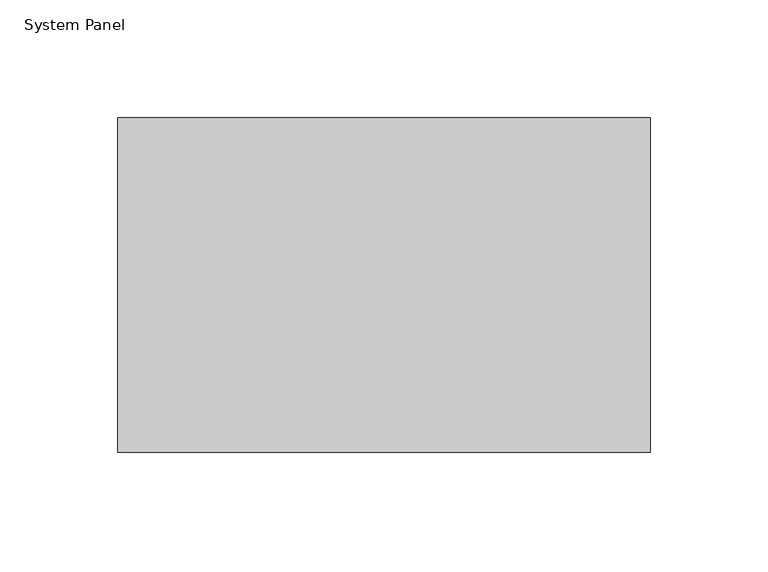
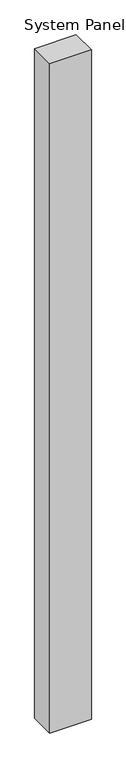
"""IFC4 building model written with IfcOpenShell, lengths in millimetres: plate geometry, System Panel : NLRS_21_CWP_hsb-vulling minerale wol 142 _gen_rsf."""

import ifcopenshell
import ifcopenshell.guid

model = None  # the IFC model being written
_history = None  # IfcOwnerHistory: only IFC2X3 demands one
_inside = {}  # id of a spatial element -> (the spatial element, [elements in it])
_under = {}  # id of a project, library or spatial element -> (it, [spatial elements below it])
_declared = {}  # id of a project -> (the project, [libraries it declares])
_typed = {}  # id of a type object -> (the type object, [elements of that type])
_made_of = {}  # id of a material, layer set ... -> (it, [elements and type objects made of it])


def new_model(schema):
    """Start an empty IFC model of exactly this schema.

    Asked for "IFC4X3", IfcOpenShell would pick the latest addendum, in which some entities
    have other attributes; the version numbers below select the first issue.
    IFC2X3 requires an IfcOwnerHistory on every rooted entity: one is made here for all.
    """
    global model, _history
    if schema == "IFC4X3":
        model = ifcopenshell.file(schema_version=(4, 3, 0, 0))
    else:
        model = ifcopenshell.file(schema=schema)
    _inside.clear()
    _under.clear()
    _declared.clear()
    _typed.clear()
    _made_of.clear()
    _history = None
    if model.schema == "IFC2X3":
        org = make("IfcOrganization", Name="unknown")
        user = make(
            "IfcPersonAndOrganization",
            ThePerson=make("IfcPerson", FamilyName="unknown"),
            TheOrganization=org,
        )
        app = make(
            "IfcApplication",
            ApplicationDeveloper=org,
            Version="unknown",
            ApplicationFullName="unknown",
            ApplicationIdentifier="unknown",
        )
        _history = make(
            "IfcOwnerHistory",
            OwningUser=user,
            OwningApplication=app,
            ChangeAction="ADDED",
            CreationDate=0,
        )
    return model


def make(cls, **values):
    """One entity of the class cls with the attributes given. An attribute that is None is left unset."""
    return model.create_entity(
        cls, **{name: value for name, value in values.items() if value is not None}
    )


def rooted(cls, **values):
    """An entity with a GlobalId (a new one), such as an element, a storey or a relation."""
    return make(cls, GlobalId=ifcopenshell.guid.new(), OwnerHistory=_history, **values)


def si_unit(unit_type, name, prefix=None):
    """IfcSIUnit, for example si_unit("LENGTHUNIT", "METRE", prefix="MILLI")."""
    return make("IfcSIUnit", UnitType=unit_type, Prefix=prefix, Name=name)


def assignment(units):
    """IfcUnitAssignment: the units of a project."""
    return None if units is None else make("IfcUnitAssignment", Units=units)


def point(xyz):
    """IfcCartesianPoint."""
    return None if xyz is None else make("IfcCartesianPoint", Coordinates=xyz)


def direction(xyz):
    """IfcDirection."""
    return None if xyz is None else make("IfcDirection", DirectionRatios=xyz)


def frame(location, z_axis=None, x_axis=None):
    """IfcAxis2Placement3D, a coordinate frame: its origin and axes. An axis left out is left unset."""
    return make(
        "IfcAxis2Placement3D",
        Location=point(location),
        Axis=direction(z_axis),
        RefDirection=direction(x_axis),
    )


def origin():
    """The frame at (0, 0, 0) with its axes left unset."""
    return frame((0.0, 0.0, 0.0))


def origin_with_axes():
    """The frame at (0, 0, 0) with the z axis (0, 0, 1) and the x axis (1, 0, 0) written out."""
    return frame((0.0, 0.0, 0.0), z_axis=(0.0, 0.0, 1.0), x_axis=(1.0, 0.0, 0.0))


def place(relative_to, where):
    """IfcLocalPlacement: puts the frame where relative to a parent placement (None: the world)."""
    return make(
        "IfcLocalPlacement", PlacementRelTo=relative_to, RelativePlacement=where
    )


def context(
    kind, dimensions, precision=None, world=None, true_north=None, identifier=None
):
    """IfcGeometricRepresentationContext, for example the 3D "Model" context."""
    return make(
        "IfcGeometricRepresentationContext",
        ContextIdentifier=identifier,
        ContextType=kind,
        CoordinateSpaceDimension=dimensions,
        Precision=precision,
        WorldCoordinateSystem=world,
        TrueNorth=true_north,
    )


def project(units=None, contexts=None):
    """IfcProject with its units and contexts."""
    return rooted(
        "IfcProject",
        Name="project",
        RepresentationContexts=contexts,
        UnitsInContext=assignment(units),
    )


def spatial(cls, under=None, at=None, **own):
    """A site, building, storey or space (cls), placed at a placement, below another one or the project."""
    s = rooted(cls, ObjectPlacement=at, **own)
    if under is not None:
        _under.setdefault(under.id(), (under, []))[1].append(s)
    return s


def polyline(points):
    """IfcPolyline through the points."""
    return make("IfcPolyline", Points=[point(p) for p in points])


def outline(outer, holes=None, kind="AREA"):
    """IfcArbitraryClosedProfileDef: a profile drawn as a closed curve; with holes, ...WithVoids."""
    if holes is None:
        return make("IfcArbitraryClosedProfileDef", ProfileType=kind, OuterCurve=outer)
    return make(
        "IfcArbitraryProfileDefWithVoids",
        ProfileType=kind,
        OuterCurve=outer,
        InnerCurves=holes,
    )


def extrude(swept, where, along, depth):
    """IfcExtrudedAreaSolid: the profile swept, set in the frame where, extruded along a direction by depth."""
    return make(
        "IfcExtrudedAreaSolid",
        SweptArea=swept,
        Position=where,
        ExtrudedDirection=direction(along),
        Depth=depth,
    )


def shape(context_of_items, identifier, shape_type, items):
    """IfcShapeRepresentation: the items that make up one representation, for example the "Body"."""
    return make(
        "IfcShapeRepresentation",
        ContextOfItems=context_of_items,
        RepresentationIdentifier=identifier,
        RepresentationType=shape_type,
        Items=items,
    )


def source(mapping_origin, context_of_items, identifier, shape_type, items):
    """IfcRepresentationMap: a shape defined once, which mapped items show again and again."""
    return make(
        "IfcRepresentationMap",
        MappingOrigin=mapping_origin,
        MappedRepresentation=shape(context_of_items, identifier, shape_type, items),
    )


def transform(
    local_origin,
    x_axis=None,
    y_axis=None,
    z_axis=None,
    scale=None,
    scale2=None,
    scale3=None,
    uniform=True,
):
    """IfcCartesianTransformationOperator3D, or its non-uniform kind. x_axis, y_axis, z_axis: its Axis1, 2, 3."""
    if uniform:
        return make(
            "IfcCartesianTransformationOperator3D",
            Axis1=direction(x_axis),
            Axis2=direction(y_axis),
            LocalOrigin=point(local_origin),
            Scale=scale,
            Axis3=direction(z_axis),
        )
    return make(
        "IfcCartesianTransformationOperator3DnonUniform",
        Axis1=direction(x_axis),
        Axis2=direction(y_axis),
        LocalOrigin=point(local_origin),
        Scale=scale,
        Axis3=direction(z_axis),
        Scale2=scale2,
        Scale3=scale3,
    )


def mapped(mapping_source, mapping_target):
    """IfcMappedItem: shows the shape of a source again, moved by a transform."""
    return make(
        "IfcMappedItem", MappingSource=mapping_source, MappingTarget=mapping_target
    )


def made_of(thing, what):
    """Note that an element or type object is made of a material, layer set ...; save() writes the relation."""
    if what is not None:
        _made_of.setdefault(what.id(), (what, []))[1].append(thing)
    return thing


def element(
    cls,
    number,
    at=None,
    inside=None,
    cuts=None,
    type_object=None,
    material=None,
    context=None,
    identifier="Body",
    shape_type=None,
    held_by="IfcProductDefinitionShape",
    body=None,
    shapes=None,
    **own,
):
    """One element of the class cls, such as IfcWall. Its Tag is "e" and its number.

    at: its placement. inside: the storey or other place that contains it. cuts: it is an
    opening in that element (IfcRelVoidsElement). A single representation is given by context,
    identifier, shape_type and body (its items); several are given by shapes. held_by: the class
    of the entity that holds the representations. save() writes the other relations.
    """
    e = rooted(cls, Tag="e%d" % number, ObjectPlacement=at, **own)
    if body is not None:
        shapes = [shape(context, identifier, shape_type, body)]
    if shapes is not None:
        e.Representation = make(held_by, Representations=shapes)
    if inside is not None:
        _inside.setdefault(inside.id(), (inside, []))[1].append(e)
    if cuts is not None:
        rooted(
            "IfcRelVoidsElement", RelatingBuildingElement=cuts, RelatedOpeningElement=e
        )
    if type_object is not None:
        _typed.setdefault(type_object.id(), (type_object, []))[1].append(e)
    return made_of(e, material)


def aggregate(whole, parts):
    """IfcRelAggregates: a whole, such as a stair, and the parts it consists of."""
    return rooted("IfcRelAggregates", RelatingObject=whole, RelatedObjects=parts)


def save(model, path):
    """Write the relations noted so far, then the file.

    IfcRelAggregates (storeys below a building ...), IfcRelContainedInSpatialStructure (elements
    in a storey), IfcRelDefinesByType, IfcRelAssociatesMaterial and IfcRelDeclares: one each for
    every whole, place, type object, material and project.
    """
    for whole, parts in _under.values():
        aggregate(whole, parts)
    for where, things in _inside.values():
        rooted(
            "IfcRelContainedInSpatialStructure",
            RelatedElements=things,
            RelatingStructure=where,
        )
    for kind, things in _typed.values():
        rooted("IfcRelDefinesByType", RelatedObjects=things, RelatingType=kind)
    for what, things in _made_of.values():
        rooted("IfcRelAssociatesMaterial", RelatedObjects=things, RelatingMaterial=what)
    for by, libraries in _declared.values():
        rooted("IfcRelDeclares", RelatingContext=by, RelatedDefinitions=libraries)
    model.write(path)


def system_panel_6e26c10f(model_context):
    return source(origin(), model_context, "Body", "SweptSolid", [
        extrude(outline(polyline([(113.0000002, -71.0), (-113.0000002, -71.0), (-113.0000002, 71.0), (113.0000002, 71.0), (113.0000002, -71.0)])), origin_with_axes(), (0.0, 0.0, 1.0), 3849.0),
    ])


if __name__ == "__main__":
    model = new_model("IFC4")
    model_context = context("Model", 3, world=origin())
    ifc_project = project(units=[si_unit("LENGTHUNIT", "METRE", prefix="MILLI")], contexts=[model_context])
    site = spatial("IfcSite", under=ifc_project)
    building = spatial("IfcBuilding", under=site)
    placement = place(None, origin())
    system_panel_shape = system_panel_6e26c10f(model_context)
    element("IfcPlate", 1, ObjectType="System Panel : NLRS_21_CWP_hsb-vulling minerale wol 142 _gen_rsf", at=placement, inside=building, context=model_context, shape_type="MappedRepresentation", body=[
        mapped(system_panel_shape, transform((0.0, 0.0, 0.0), x_axis=(1.0, 0.0, 0.0), y_axis=(0.0, 1.0, 0.0), z_axis=(0.0, 0.0, 1.0))),
    ])
    save(model, "model.ifc")

# Revit data of these elements
# Type "System Panel : NLRS_21_CWP_hsb-vulling minerale wol 142 _gen_rsf"
#   Export Type to IFC As = "IfcWall"
#   Type IfcGUID = "07M7mRoiH1CR8m_RSKIwpC"
#   Assembly Code = "21.23"
# Element 1 (IfcPlate, "System Panel : NLRS_21_CWP_hsb-vulling minerale wol 142 _gen_rsf")
#   Materials on its faces: "NLRS_m1_isolatie minerale wol_gen_rsf"
# Materials
#   "NLRS_m1_isolatie minerale wol_gen_rsf": class "M - Anorganische materialen", colour RGB 200 200 140, transparency 0, Keynote = "m1", Manufacturer = "Revit Standards Foundation", URL = "www.revitstandards.org", Description = "isolatie minerale wol", Cost = 0
